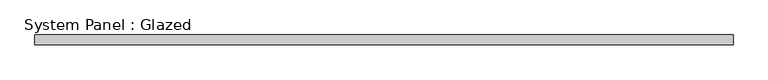
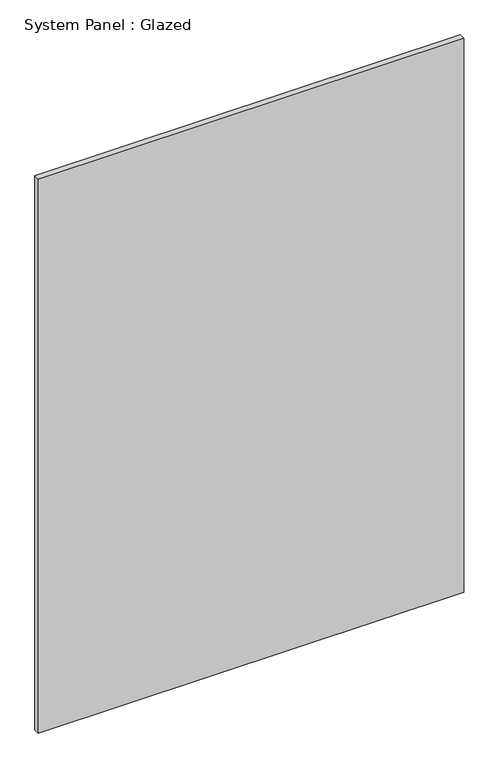
"""IFC4 building model written with IfcOpenShell, lengths in millimetres: plate geometry, System Panel : Glazed."""

from ifc_helpers import new_model, si_unit, origin, origin_with_axes, place, context, project, spatial, polyline, outline, extrude, source, transform, mapped, element, save


def system_panel_glazed_3dade0f0(model_context):
    return source(origin(), model_context, "Body", "SweptSolid", [
        extrude(outline(polyline([(890.0, 24.5), (-890.0, 24.5), (-890.0, 49.5), (890.0, 49.5), (890.0, 24.5)])), origin_with_axes(), (0.0, 0.0, 1.0), 2450.0),
    ])


if __name__ == "__main__":
    model = new_model("IFC4")
    model_context = context("Model", 3, world=origin())
    ifc_project = project(units=[si_unit("LENGTHUNIT", "METRE", prefix="MILLI")], contexts=[model_context])
    site = spatial("IfcSite", under=ifc_project)
    building = spatial("IfcBuilding", under=site)
    placement = place(None, origin())
    system_panel_glazed_shape = system_panel_glazed_3dade0f0(model_context)
    element("IfcPlate", 1, ObjectType="System Panel : Glazed", at=placement, inside=building, context=model_context, shape_type="MappedRepresentation", body=[
        mapped(system_panel_glazed_shape, transform((0.0, 0.0, 0.0), x_axis=(1.0, 0.0, 0.0), y_axis=(0.0, 1.0, 0.0), z_axis=(0.0, 0.0, 1.0))),
    ])
    save(model, "model.ifc")

# Revit data of these elements
# Type "System Panel : Glazed"
#   Keynote = "H11"
#   Construction Type Id = "GSP4R"
#   Analytic Construction = "1/8 in Pilkington single glazing"
#   Visual Light Transmittance = 0.9
#   Solar Heat Gain Coefficient = 0.86
#   Heat Transfer Coefficient (U) = 6.7069 W/(m²·K)
# Element 1 (IfcPlate, "System Panel : Glazed")
#   Materials on its faces: "Glass"
# Materials
#   "Glass": class "Glass", colour RGB 0 128 192, transparency 0.9, Description = "Soda Lime Glass", Cost = 0
